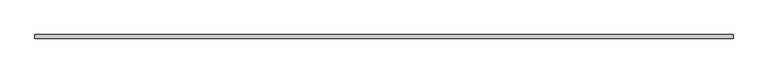
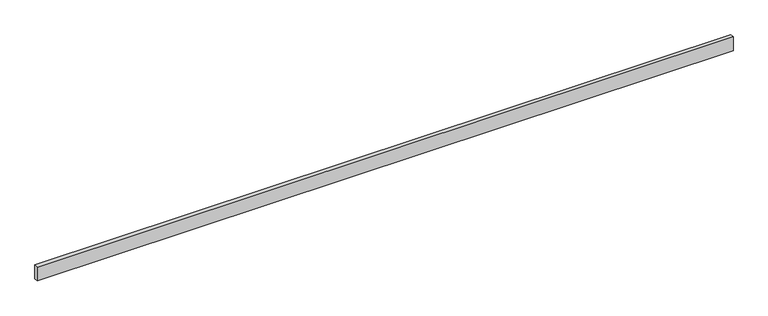
"""IFC4 building model written with IfcOpenShell, lengths in millimetres: proxy geometry, Generic Models 7:Generic Models 1:337419:Generic Models 1:337419 : Generic Models 7:Generic Models 1:337419:39 : Generic Models 7:Generic Models 1:337419:Generic Models 1:337419 : Generic Models 7:Generic Models 1:337419:301336."""

from ifc_helpers import new_model, si_unit, frame, origin, place, context, project, spatial, polyline, outline, extrude, source, transform, mapped, element, save


def generic_models_23f2a1a1(model_context):
    return source(origin(), model_context, "Body", "SweptSolid", [
        extrude(outline(polyline([(596182.8367242, -536531.8913358), (596182.8367242, -536557.2913358), (591306.0367242, -536557.2913358), (591306.0367242, -536531.8913358), (596182.8367242, -536531.8913358)])), frame((0.0, 0.0, 3605.0140625), z_axis=(0.0, 0.0, 1.0), x_axis=(1.0, 0.0, 0.0)), (0.0, 0.0, 1.0), 101.6),
    ])


if __name__ == "__main__":
    model = new_model("IFC4")
    model_context = context("Model", 3, world=origin())
    ifc_project = project(units=[si_unit("LENGTHUNIT", "METRE", prefix="MILLI")], contexts=[model_context])
    site = spatial("IfcSite", under=ifc_project)
    building = spatial("IfcBuilding", under=site)
    placement = place(None, origin())
    generic_models_shape = generic_models_23f2a1a1(model_context)
    element("IfcBuildingElementProxy", 1, Name="Generic Models 7:Generic Models 1:337419:Generic Models 1:337419 : Generic Models 7:Generic Models 1:337419:39 : Generic Models 7:Generic Models 1:337419:Generic Models 1:337419 : Generic Models 7:Generic Models 1:337419:301336", ObjectType="Generic Models 7:Generic Models 1:337419:Generic Models 1:337419 : Generic Models 7:Generic Models 1:337419:39 : Generic Models 7:Generic Models 1:337419:Generic Models 1:337419 : Generic Models 7:Generic Models 1:337419:301336", at=placement, inside=building, context=model_context, shape_type="MappedRepresentation", body=[
        mapped(generic_models_shape, transform((0.0, 0.0, 0.0), x_axis=(1.0, 0.0, 0.0), y_axis=(0.0, 1.0, 0.0), z_axis=(0.0, 0.0, 1.0))),
    ])
    save(model, "model.ifc")

# Revit data of these elements
# Type "Generic Models 7:Generic Models 1:337419:Generic Models 1:337419 : Generic Models 7:Generic Models 1:337419:39 : Generic Models 7:Generic Models 1:337419:Generic Models 1:337419 : Generic Models 7:Generic Models 1:337419:301336"
#   NameOverride = "Generic Models 7:Generic Models 1:337419:Generic Models 1:337419 : Generic Models 7:Generic Models 1:337419:301336"
#   ObjectTypeOverride = "Generic Models 1:337419 : Generic Models 7:Generic Models 1:337419"
#   Reference = "Generic Models 1"
#   Tag = "301336"
# Element 1 (IfcBuildingElementProxy, "Generic Models 7:Generic Models 1:337419:Generic Models 1:337419 : Generic Models 7:Generic Models 1:337419:39 : Generic Models 7:Generic Models 1:337419:Generic Models 1:337419 : Generic Models 7:Generic Models 1:337419:301336")
#   Materials on its faces: "RIGID INSULATION AT GIRTS/JAMB - (CLASS A FLAME SPREAD)"
# Materials
#   "RIGID INSULATION AT GIRTS/JAMB - (CLASS A FLAME SPREAD)": class "Unassigned", colour RGB 205 188 106, transparency 0, Cost = 0
